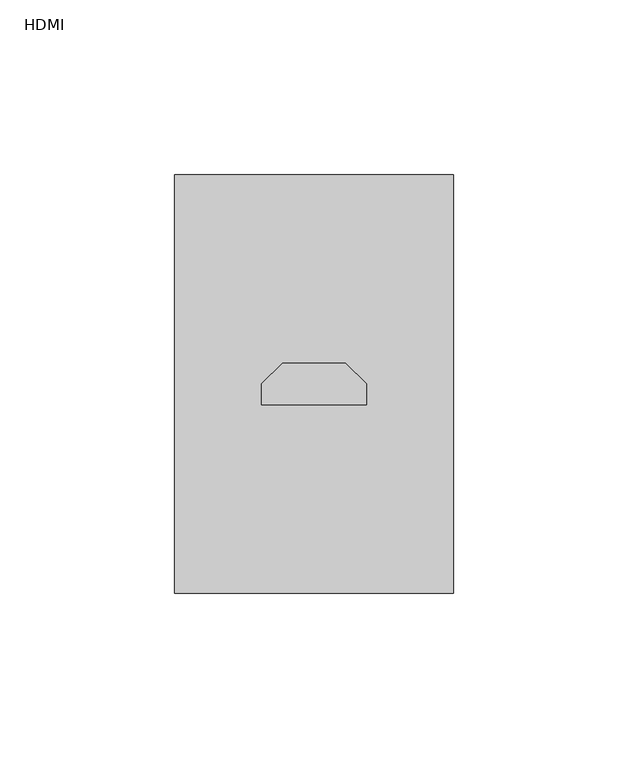
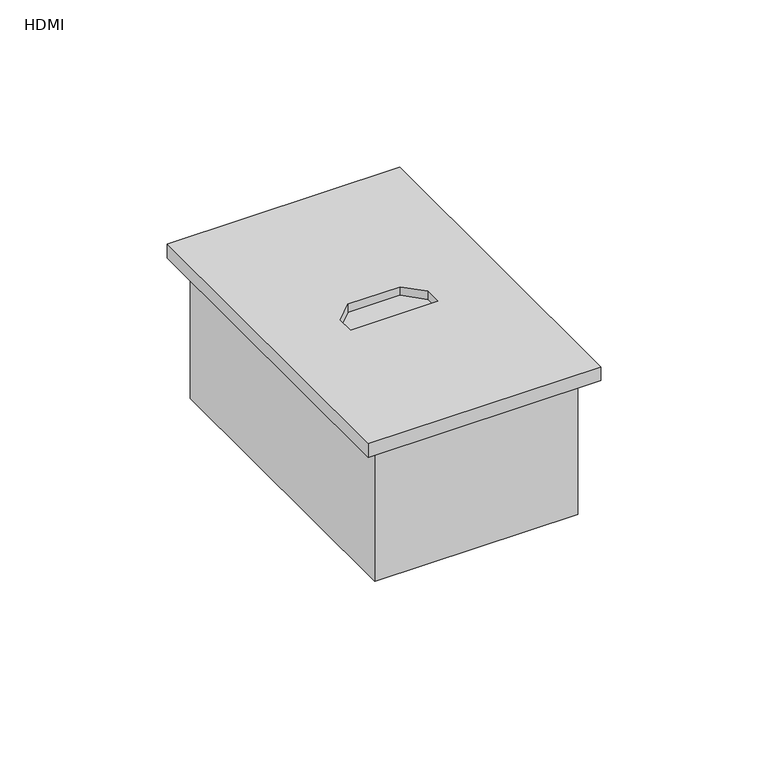
"""IFC4 building model written with IfcOpenShell, lengths in millimetres: proxy geometry, CAIXA VERTICE V7 : HDMI."""

from ifc_helpers import new_model, si_unit, origin, place, context, project, spatial, faceted_brep, source, transform, mapped, element, save


def hdmi_62cd6cdd(model_context):
    return source(origin(), model_context, "Body", "Brep", [
        faceted_brep([(33.0, 1047.0, -48.0), (33.0, 1153.0, -48.0), (-33.0, 1153.0, -48.0), (-33.0, 1047.0, -48.0), (35.0, 1155.0, -50.0), (35.0, 1045.0, -50.0), (-35.0, 1045.0, -50.0), (-35.0, 1155.0, -50.0), (-35.0, 1155.0, 0.0), (35.0, 1155.0, 0.0), (-35.0, 1045.0, 0.0), (35.0, 1045.0, 0.0), (33.0, 1153.0, 0.0), (33.0, 1047.0, 0.0), (-33.0, 1047.0, 0.0), (-33.0, 1153.0, 0.0)], [[[0, 1, 2, 3]], [[4, 5, 6, 7]], [[4, 7, 8, 9]], [[8, 7, 6, 10]], [[10, 6, 5, 11]], [[11, 5, 4, 9]], [[9, 8, 10, 11], [12, 13, 14, 15]], [[13, 12, 1, 0]], [[14, 13, 0, 3]], [[15, 14, 3, 2]], [[12, 15, 2, 1]]]),
        faceted_brep([(40.0, 1160.0, 5.0), (-40.0, 1160.0, 5.0), (-40.0, 1040.0, 5.0), (40.0, 1040.0, 5.0), (-15.0, 1094.0, 5.0), (-15.0, 1100.0, 5.0), (-9.0, 1106.0, 5.0), (9.0, 1106.0, 5.0), (15.0, 1100.0, 5.0), (15.0, 1094.0, 5.0), (-40.0, 1160.0, 0.0), (40.0, 1160.0, 0.0), (40.0, 1040.0, 0.0), (-40.0, 1040.0, 0.0), (-15.0, 1094.0, 2.0), (-15.0, 1100.0, 2.0), (-9.0, 1106.0, 2.0), (9.0, 1106.0, 2.0), (15.0, 1100.0, 2.0), (15.0, 1094.0, 2.0)], [[[0, 1, 2, 3], [4, 5, 6, 7, 8, 9]], [[10, 11, 12, 13]], [[1, 0, 11, 10]], [[2, 1, 10, 13]], [[3, 2, 13, 12]], [[0, 3, 12, 11]], [[14, 15, 5, 4]], [[15, 16, 6, 5]], [[17, 18, 8, 7]], [[17, 16, 15, 14, 19, 18]], [[16, 17, 7, 6]], [[18, 19, 9, 8]], [[19, 14, 4, 9]]]),
    ])


if __name__ == "__main__":
    model = new_model("IFC4")
    model_context = context("Model", 3, world=origin())
    ifc_project = project(units=[si_unit("LENGTHUNIT", "METRE", prefix="MILLI")], contexts=[model_context])
    site = spatial("IfcSite", under=ifc_project)
    building = spatial("IfcBuilding", under=site)
    placement = place(None, origin())
    hdmi_shape = hdmi_62cd6cdd(model_context)
    element("IfcBuildingElementProxy", 1, Name="CAIXA VERTICE V7 : HDMI", ObjectType="CAIXA VERTICE V7 : HDMI", at=placement, inside=building, context=model_context, shape_type="MappedRepresentation", body=[
        mapped(hdmi_shape, transform((0.0, 0.0, 0.0), x_axis=(1.0, 0.0, 0.0), y_axis=(0.0, 1.0, 0.0), z_axis=(0.0, 0.0, 1.0))),
    ])
    save(model, "model.ifc")

# Revit data of these elements
# Type "CAIXA VERTICE V7 : HDMI"
#   URL = "www.facebook.com/verticetreinamentos"
#   SEÇÃO [instance default] = ""
#   Rotação [instance default] = 0.00°
#   LARGURA DA TAMPA = 0.08 m
#   BORDA = 0.01 m
#   ALTURA DE INSTALAÇÃO [instance default] = 1.10 m
#   Distância Anotação [instance default] = 0.0015 m
#   ALTURA DA TAMPA = 0.12 m
#   Vertical [instance default] = yes
#   VER SEÇÃO [instance default] = yes
#   SHADE ESQ [instance default] = no
#   SHADE DIR [instance default] = yes
#   HORIZONTAL [instance default] = no
#   ANDAR COM A LEGENDA [instance default] = 0
#   Material Tampa [instance default] = Plástico, branco opaco
#   Caixa = element 1798549
#   Anotação = element 1798548
#   Default Elevation = 0
# Element 1 (IfcBuildingElementProxy, "CAIXA VERTICE V7 : HDMI")
#   Materials on its faces: "Plástico, branco opaco"
# Materials
#   "Plástico, branco opaco": class "Plástico", colour RGB 120 120 120, transparency 0, Description = "Plastic, generic, opaque white", Cost = 0
